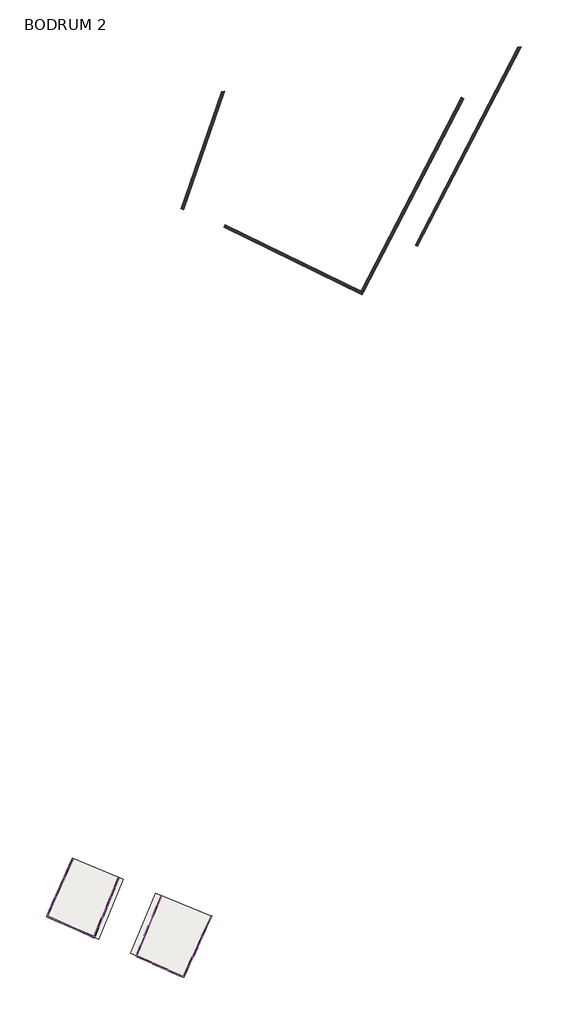
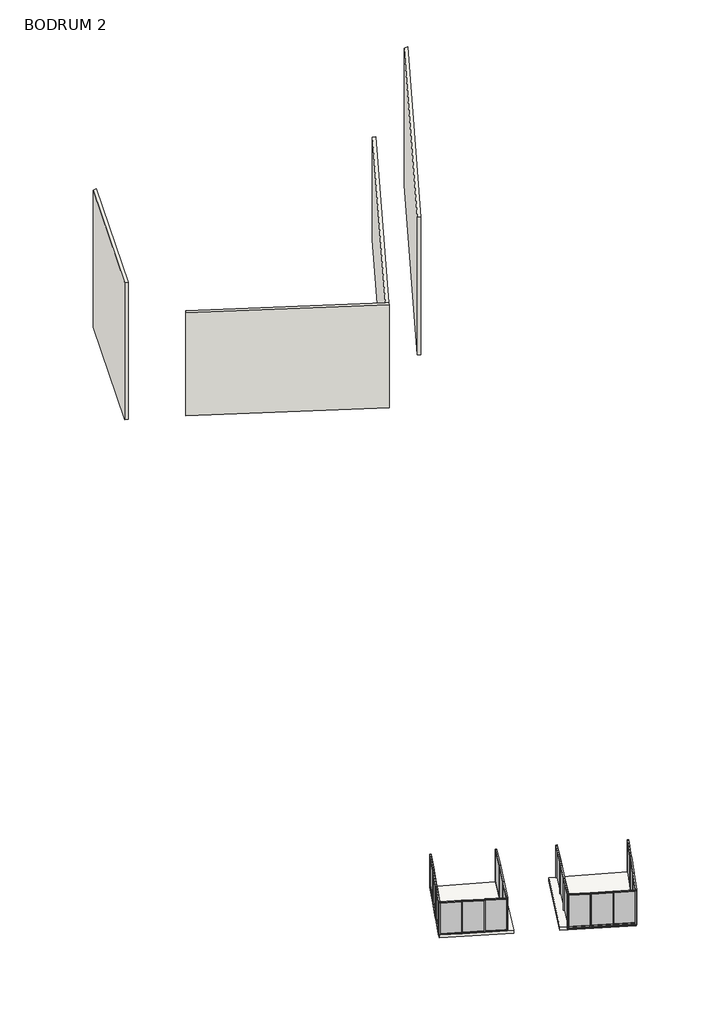
# One storey: 60 members, 18 plates, 4 walls, 1 slab.
"""IFC4 building model written with IfcOpenShell, lengths in millimetres."""

import ifcopenshell
import ifcopenshell.guid

model = None  # the IFC model being written
_history = None  # IfcOwnerHistory: only IFC2X3 demands one
_inside = {}  # id of a spatial element -> (the spatial element, [elements in it])
_under = {}  # id of a project, library or spatial element -> (it, [spatial elements below it])
_declared = {}  # id of a project -> (the project, [libraries it declares])
_typed = {}  # id of a type object -> (the type object, [elements of that type])
_made_of = {}  # id of a material, layer set ... -> (it, [elements and type objects made of it])


def new_model(schema):
    """Start an empty IFC model of exactly this schema.

    Asked for "IFC4X3", IfcOpenShell would pick the latest addendum, in which some entities
    have other attributes; the version numbers below select the first issue.
    IFC2X3 requires an IfcOwnerHistory on every rooted entity: one is made here for all.
    """
    global model, _history
    if schema == "IFC4X3":
        model = ifcopenshell.file(schema_version=(4, 3, 0, 0))
    else:
        model = ifcopenshell.file(schema=schema)
    _inside.clear()
    _under.clear()
    _declared.clear()
    _typed.clear()
    _made_of.clear()
    _history = None
    if model.schema == "IFC2X3":
        org = make("IfcOrganization", Name="unknown")
        user = make(
            "IfcPersonAndOrganization",
            ThePerson=make("IfcPerson", FamilyName="unknown"),
            TheOrganization=org,
        )
        app = make(
            "IfcApplication",
            ApplicationDeveloper=org,
            Version="unknown",
            ApplicationFullName="unknown",
            ApplicationIdentifier="unknown",
        )
        _history = make(
            "IfcOwnerHistory",
            OwningUser=user,
            OwningApplication=app,
            ChangeAction="ADDED",
            CreationDate=0,
        )
    return model


def make(cls, **values):
    """One entity of the class cls with the attributes given. An attribute that is None is left unset."""
    return model.create_entity(
        cls, **{name: value for name, value in values.items() if value is not None}
    )


def rooted(cls, **values):
    """An entity with a GlobalId (a new one), such as an element, a storey or a relation."""
    return make(cls, GlobalId=ifcopenshell.guid.new(), OwnerHistory=_history, **values)


def si_unit(unit_type, name, prefix=None):
    """IfcSIUnit, for example si_unit("LENGTHUNIT", "METRE", prefix="MILLI")."""
    return make("IfcSIUnit", UnitType=unit_type, Prefix=prefix, Name=name)


def assignment(units):
    """IfcUnitAssignment: the units of a project."""
    return None if units is None else make("IfcUnitAssignment", Units=units)


def point(xyz):
    """IfcCartesianPoint."""
    return None if xyz is None else make("IfcCartesianPoint", Coordinates=xyz)


def direction(xyz):
    """IfcDirection."""
    return None if xyz is None else make("IfcDirection", DirectionRatios=xyz)


def frame(location, z_axis=None, x_axis=None):
    """IfcAxis2Placement3D, a coordinate frame: its origin and axes. An axis left out is left unset."""
    return make(
        "IfcAxis2Placement3D",
        Location=point(location),
        Axis=direction(z_axis),
        RefDirection=direction(x_axis),
    )


def origin():
    """The frame at (0, 0, 0) with its axes left unset."""
    return frame((0.0, 0.0, 0.0))


def origin_with_axes():
    """The frame at (0, 0, 0) with the z axis (0, 0, 1) and the x axis (1, 0, 0) written out."""
    return frame((0.0, 0.0, 0.0), z_axis=(0.0, 0.0, 1.0), x_axis=(1.0, 0.0, 0.0))


def place(relative_to, where):
    """IfcLocalPlacement: puts the frame where relative to a parent placement (None: the world)."""
    return make(
        "IfcLocalPlacement", PlacementRelTo=relative_to, RelativePlacement=where
    )


def context(
    kind, dimensions, precision=None, world=None, true_north=None, identifier=None
):
    """IfcGeometricRepresentationContext, for example the 3D "Model" context."""
    return make(
        "IfcGeometricRepresentationContext",
        ContextIdentifier=identifier,
        ContextType=kind,
        CoordinateSpaceDimension=dimensions,
        Precision=precision,
        WorldCoordinateSystem=world,
        TrueNorth=true_north,
    )


def project(units=None, contexts=None):
    """IfcProject with its units and contexts."""
    return rooted(
        "IfcProject",
        Name="project",
        RepresentationContexts=contexts,
        UnitsInContext=assignment(units),
    )


def spatial(cls, under=None, at=None, **own):
    """A site, building, storey or space (cls), placed at a placement, below another one or the project."""
    s = rooted(cls, ObjectPlacement=at, **own)
    if under is not None:
        _under.setdefault(under.id(), (under, []))[1].append(s)
    return s


def polyline(points):
    """IfcPolyline through the points."""
    return make("IfcPolyline", Points=[point(p) for p in points])


def outline(outer, holes=None, kind="AREA"):
    """IfcArbitraryClosedProfileDef: a profile drawn as a closed curve; with holes, ...WithVoids."""
    if holes is None:
        return make("IfcArbitraryClosedProfileDef", ProfileType=kind, OuterCurve=outer)
    return make(
        "IfcArbitraryProfileDefWithVoids",
        ProfileType=kind,
        OuterCurve=outer,
        InnerCurves=holes,
    )


def extrude(swept, where, along, depth):
    """IfcExtrudedAreaSolid: the profile swept, set in the frame where, extruded along a direction by depth."""
    return make(
        "IfcExtrudedAreaSolid",
        SweptArea=swept,
        Position=where,
        ExtrudedDirection=direction(along),
        Depth=depth,
    )


def faces_of(points, faces, orient=None, outer=None):
    """IfcFace entities. A face is a list of loops; a loop is a list of indices into points, from 0.

    orient and outer hold one flag for each loop. By default every Orientation is true, the
    first loop of a face is its IfcFaceOuterBound and the others are IfcFaceBound.
    """
    made = []
    for i, loops in enumerate(faces):
        bounds = []
        for j, loop in enumerate(loops):
            is_outer = j == 0 if outer is None else outer[i][j]
            bounds.append(
                make(
                    "IfcFaceOuterBound" if is_outer else "IfcFaceBound",
                    Bound=make("IfcPolyLoop", Polygon=[points[k] for k in loop]),
                    Orientation=True if orient is None else orient[i][j],
                )
            )
        made.append(make("IfcFace", Bounds=bounds))
    return made


def faceted_brep(points, faces, orient=None, outer=None, voids=None):
    """IfcFacetedBrep: a solid bounded by flat faces; with voids (closed shells), ...WithVoids."""
    shared = [point(p) for p in points]
    hull = make("IfcClosedShell", CfsFaces=faces_of(shared, faces, orient, outer))
    if voids is None:
        return make("IfcFacetedBrep", Outer=hull)
    return make(
        "IfcFacetedBrepWithVoids",
        Outer=hull,
        Voids=[
            make(cls, CfsFaces=faces_of(shared, fs, o, b)) for cls, fs, o, b in voids
        ],
    )


def shape(context_of_items, identifier, shape_type, items):
    """IfcShapeRepresentation: the items that make up one representation, for example the "Body"."""
    return make(
        "IfcShapeRepresentation",
        ContextOfItems=context_of_items,
        RepresentationIdentifier=identifier,
        RepresentationType=shape_type,
        Items=items,
    )


def source(mapping_origin, context_of_items, identifier, shape_type, items):
    """IfcRepresentationMap: a shape defined once, which mapped items show again and again."""
    return make(
        "IfcRepresentationMap",
        MappingOrigin=mapping_origin,
        MappedRepresentation=shape(context_of_items, identifier, shape_type, items),
    )


def transform(
    local_origin,
    x_axis=None,
    y_axis=None,
    z_axis=None,
    scale=None,
    scale2=None,
    scale3=None,
    uniform=True,
):
    """IfcCartesianTransformationOperator3D, or its non-uniform kind. x_axis, y_axis, z_axis: its Axis1, 2, 3."""
    if uniform:
        return make(
            "IfcCartesianTransformationOperator3D",
            Axis1=direction(x_axis),
            Axis2=direction(y_axis),
            LocalOrigin=point(local_origin),
            Scale=scale,
            Axis3=direction(z_axis),
        )
    return make(
        "IfcCartesianTransformationOperator3DnonUniform",
        Axis1=direction(x_axis),
        Axis2=direction(y_axis),
        LocalOrigin=point(local_origin),
        Scale=scale,
        Axis3=direction(z_axis),
        Scale2=scale2,
        Scale3=scale3,
    )


def mapped(mapping_source, mapping_target):
    """IfcMappedItem: shows the shape of a source again, moved by a transform."""
    return make(
        "IfcMappedItem", MappingSource=mapping_source, MappingTarget=mapping_target
    )


def made_of(thing, what):
    """Note that an element or type object is made of a material, layer set ...; save() writes the relation."""
    if what is not None:
        _made_of.setdefault(what.id(), (what, []))[1].append(thing)
    return thing


def element(
    cls,
    number,
    at=None,
    inside=None,
    cuts=None,
    type_object=None,
    material=None,
    context=None,
    identifier="Body",
    shape_type=None,
    held_by="IfcProductDefinitionShape",
    body=None,
    shapes=None,
    **own,
):
    """One element of the class cls, such as IfcWall. Its Tag is "e" and its number.

    at: its placement. inside: the storey or other place that contains it. cuts: it is an
    opening in that element (IfcRelVoidsElement). A single representation is given by context,
    identifier, shape_type and body (its items); several are given by shapes. held_by: the class
    of the entity that holds the representations. save() writes the other relations.
    """
    e = rooted(cls, Tag="e%d" % number, ObjectPlacement=at, **own)
    if body is not None:
        shapes = [shape(context, identifier, shape_type, body)]
    if shapes is not None:
        e.Representation = make(held_by, Representations=shapes)
    if inside is not None:
        _inside.setdefault(inside.id(), (inside, []))[1].append(e)
    if cuts is not None:
        rooted(
            "IfcRelVoidsElement", RelatingBuildingElement=cuts, RelatedOpeningElement=e
        )
    if type_object is not None:
        _typed.setdefault(type_object.id(), (type_object, []))[1].append(e)
    return made_of(e, material)


def aggregate(whole, parts):
    """IfcRelAggregates: a whole, such as a stair, and the parts it consists of."""
    return rooted("IfcRelAggregates", RelatingObject=whole, RelatedObjects=parts)


def save(model, path):
    """Write the relations noted so far, then the file.

    IfcRelAggregates (storeys below a building ...), IfcRelContainedInSpatialStructure (elements
    in a storey), IfcRelDefinesByType, IfcRelAssociatesMaterial and IfcRelDeclares: one each for
    every whole, place, type object, material and project.
    """
    for whole, parts in _under.values():
        aggregate(whole, parts)
    for where, things in _inside.values():
        rooted(
            "IfcRelContainedInSpatialStructure",
            RelatedElements=things,
            RelatingStructure=where,
        )
    for kind, things in _typed.values():
        rooted("IfcRelDefinesByType", RelatedObjects=things, RelatingType=kind)
    for what, things in _made_of.values():
        rooted("IfcRelAssociatesMaterial", RelatedObjects=things, RelatingMaterial=what)
    for by, libraries in _declared.values():
        rooted("IfcRelDeclares", RelatingContext=by, RelatedDefinitions=libraries)
    model.write(path)


def rectangular_mullion_65_x_125mm_rectangular_245190dc(model_context):
    return source(origin(), model_context, "Body", "SweptSolid", [
        extrude(outline(polyline([(0.0, 62.5), (0.0, -62.5), (-65.0, -62.5), (-65.0, 62.5), (0.0, 62.5)])), frame((0.0, 0.0, -2244.830414), z_axis=(0.0, 0.0, 1.0), x_axis=(1.0, 0.0, 0.0)), (0.0, 0.0, 1.0), 2244.830414),
    ])


def rectangular_mullion_65_x_125mm_rectangular_478791df(model_context):
    return source(origin(), model_context, "Body", "SweptSolid", [
        extrude(outline(polyline([(0.0, 62.5), (0.0, -62.5), (-65.0, -62.5), (-65.0, 62.5), (0.0, 62.5)])), frame((0.0, 0.0, -2277.3304137), z_axis=(0.0, 0.0, 1.0), x_axis=(1.0, 0.0, 0.0)), (0.0, 0.0, 1.0), 2277.3304137),
    ])


def rectangular_mullion_65_x_125mm_rectangular_36adfa9f(model_context):
    return source(origin(), model_context, "Body", "SweptSolid", [
        extrude(outline(polyline([(0.0, 62.5), (0.0, -62.5), (-65.0, -62.5), (-65.0, 62.5), (0.0, 62.5)])), frame((0.0, 0.0, -1809.1666668), z_axis=(0.0, 0.0, 1.0), x_axis=(1.0, 0.0, 0.0)), (0.0, 0.0, 1.0), 1809.1666668),
    ])


def rectangular_mullion_65_x_125mm_rectangular_c7ba065f(model_context):
    return source(origin(), model_context, "Body", "SweptSolid", [
        extrude(outline(polyline([(0.0, 62.5), (0.0, -62.5), (-65.0, -62.5), (-65.0, 62.5), (0.0, 62.5)])), frame((0.0, 0.0, -1841.6666665), z_axis=(0.0, 0.0, 1.0), x_axis=(1.0, 0.0, 0.0)), (0.0, 0.0, 1.0), 1841.6666665),
    ])


def rectangular_mullion_65_x_125mm_rectangular_4f7d984b(model_context):
    return source(origin(), model_context, "Body", "SweptSolid", [
        extrude(outline(polyline([(0.0, 62.5), (0.0, -62.5), (-65.0, -62.5), (-65.0, 62.5), (0.0, 62.5)])), frame((0.0, 0.0, -2291.9433297), z_axis=(0.0, 0.0, 1.0), x_axis=(1.0, 0.0, 0.0)), (0.0, 0.0, 1.0), 2291.9433297),
    ])


def rectangular_mullion_65_x_125mm_rectangular_64dbaea3(model_context):
    return source(origin(), model_context, "Body", "SweptSolid", [
        extrude(outline(polyline([(0.0, 62.5), (0.0, -62.5), (-65.0, -62.5), (-65.0, 62.5), (0.0, 62.5)])), frame((0.0, 0.0, -2324.4433294), z_axis=(0.0, 0.0, 1.0), x_axis=(1.0, 0.0, 0.0)), (0.0, 0.0, 1.0), 2324.4433294),
    ])


def rectangular_mullion_65_x_125mm_rectangular_bddaf145(model_context):
    return source(origin(), model_context, "Body", "SweptSolid", [
        extrude(outline(polyline([(32.5, 62.5), (32.5, -62.5), (-32.5, -62.5), (-32.5, 62.5), (32.5, 62.5)])), frame((0.0, 0.0, -3300.0), z_axis=(0.0, 0.0, 1.0), x_axis=(1.0, 0.0, 0.0)), (0.0, 0.0, 1.0), 3300.0),
    ])


def rectangular_mullion_65_x_125mm_rectangular_6bff5ffe(model_context):
    return source(origin(), model_context, "Body", "SweptSolid", [
        extrude(outline(polyline([(0.0, 62.5), (0.0, -62.5), (-65.0, -62.5), (-65.0, 62.5), (0.0, 62.5)])), frame((0.0, 0.0, -3300.0), z_axis=(0.0, 0.0, 1.0), x_axis=(1.0, 0.0, 0.0)), (0.0, 0.0, 1.0), 3300.0),
    ])


def rectangular_mullion_65_x_125mm_rectangular_eddbc5d6(model_context):
    return source(origin(), model_context, "Body", "SweptSolid", [
        extrude(outline(polyline([(0.0, 62.5), (0.0, -62.5), (-65.0, -62.5), (-65.0, 62.5), (0.0, 62.5)])), frame((0.0, 0.0, -2323.142254), z_axis=(0.0, 0.0, 1.0), x_axis=(1.0, 0.0, 0.0)), (0.0, 0.0, 1.0), 2323.142254),
    ])


def rectangular_mullion_65_x_125mm_rectangular_617b4e42(model_context):
    return source(origin(), model_context, "Body", "SweptSolid", [
        extrude(outline(polyline([(0.0, 62.5), (0.0, -62.5), (-65.0, -62.5), (-65.0, 62.5), (0.0, 62.5)])), frame((0.0, 0.0, -2355.6422537), z_axis=(0.0, 0.0, 1.0), x_axis=(1.0, 0.0, 0.0)), (0.0, 0.0, 1.0), 2355.6422537),
    ])


def rectangular_mullion_65_x_125mm_rectangular_c6a61499(model_context):
    return source(origin(), model_context, "Body", "SweptSolid", [
        extrude(outline(polyline([(32.5, 62.5), (32.5, -62.5), (-32.5, -62.5), (-32.5, 62.5), (32.5, 62.5)])), frame((0.0, 0.0, -3500.0), z_axis=(0.0, 0.0, 1.0), x_axis=(1.0, 0.0, 0.0)), (0.0, 0.0, 1.0), 3500.0),
    ])


def rectangular_mullion_65_x_125mm_rectangular_efb59fec(model_context):
    return source(origin(), model_context, "Body", "SweptSolid", [
        extrude(outline(polyline([(0.0, 62.5), (0.0, -62.5), (-65.0, -62.5), (-65.0, 62.5), (0.0, 62.5)])), frame((0.0, 0.0, -3500.0), z_axis=(0.0, 0.0, 1.0), x_axis=(1.0, 0.0, 0.0)), (0.0, 0.0, 1.0), 3500.0),
    ])


def rectangular_mullion_65_x_125mm_rectangular_567d2977(model_context):
    return source(origin(), model_context, "Body", "SweptSolid", [
        extrude(outline(polyline([(0.0, 62.5), (0.0, -62.5), (-65.0, -62.5), (-65.0, 62.5), (0.0, 62.5)])), frame((0.0, 0.0, -1811.8827626), z_axis=(0.0, 0.0, 1.0), x_axis=(1.0, 0.0, 0.0)), (0.0, 0.0, 1.0), 1811.8827626),
    ])


def rectangular_mullion_65_x_125mm_rectangular_abf36099(model_context):
    return source(origin(), model_context, "Body", "SweptSolid", [
        extrude(outline(polyline([(0.0, 62.5), (0.0, -62.5), (-65.0, -62.5), (-65.0, 62.5), (0.0, 62.5)])), frame((0.0, 0.0, -1844.3827623), z_axis=(0.0, 0.0, 1.0), x_axis=(1.0, 0.0, 0.0)), (0.0, 0.0, 1.0), 1844.3827623),
    ])


def rectangular_mullion_65_x_125mm_rectangular_944d97ce(model_context):
    return source(origin(), model_context, "Body", "SweptSolid", [
        extrude(outline(polyline([(0.0, 62.5), (0.0, -62.5), (-65.0, -62.5), (-65.0, 62.5), (0.0, 62.5)])), frame((0.0, 0.0, -2373.0683182), z_axis=(0.0, 0.0, 1.0), x_axis=(1.0, 0.0, 0.0)), (0.0, 0.0, 1.0), 2373.0683182),
    ])


def rectangular_mullion_65_x_125mm_rectangular_8233692a(model_context):
    return source(origin(), model_context, "Body", "SweptSolid", [
        extrude(outline(polyline([(0.0, 62.5), (0.0, -62.5), (-65.0, -62.5), (-65.0, 62.5), (0.0, 62.5)])), frame((0.0, 0.0, -2405.5683179), z_axis=(0.0, 0.0, 1.0), x_axis=(1.0, 0.0, 0.0)), (0.0, 0.0, 1.0), 2405.5683179),
    ])


def system_panel_glazed_19379390(model_context):
    return source(origin(), model_context, "Body", "SweptSolid", [
        extrude(outline(polyline([(1122.415207, 24.5), (-1122.415207, 24.5), (-1122.415207, 49.5), (1122.415207, 49.5), (1122.415207, 24.5)])), origin_with_axes(), (0.0, 0.0, 1.0), 3170.0),
    ])


def system_panel_glazed_0a1ee489(model_context):
    return source(origin(), model_context, "Body", "SweptSolid", [
        extrude(outline(polyline([(1138.6652068, 24.5), (-1138.6652068, 24.5), (-1138.6652068, 49.5), (1138.6652068, 49.5), (1138.6652068, 24.5)])), origin_with_axes(), (0.0, 0.0, 1.0), 3170.0),
    ])


def system_panel_glazed_d1c08d78(model_context):
    return source(origin(), model_context, "Body", "SweptSolid", [
        extrude(outline(polyline([(904.5833334, 24.5), (-904.5833334, 24.5), (-904.5833334, 49.5), (904.5833334, 49.5), (904.5833334, 24.5)])), origin_with_axes(), (0.0, 0.0, 1.0), 3170.0),
    ])


def system_panel_glazed_7daaf864(model_context):
    return source(origin(), model_context, "Body", "SweptSolid", [
        extrude(outline(polyline([(920.8333332, 24.5), (-920.8333332, 24.5), (-920.8333332, 49.5), (920.8333332, 49.5), (920.8333332, 24.5)])), origin_with_axes(), (0.0, 0.0, 1.0), 3170.0),
    ])


def system_panel_glazed_4d4608c9(model_context):
    return source(origin(), model_context, "Body", "SweptSolid", [
        extrude(outline(polyline([(1145.9716649, 24.5), (-1145.9716649, 24.5), (-1145.9716649, 49.5), (1145.9716649, 49.5), (1145.9716649, 24.5)])), origin_with_axes(), (0.0, 0.0, 1.0), 3170.0),
    ])


def system_panel_glazed_4b2262bb(model_context):
    return source(origin(), model_context, "Body", "SweptSolid", [
        extrude(outline(polyline([(1162.2216647, 24.5), (-1162.2216647, 24.5), (-1162.2216647, 49.5), (1162.2216647, 49.5), (1162.2216647, 24.5)])), origin_with_axes(), (0.0, 0.0, 1.0), 3170.0),
    ])


def system_panel_glazed_6ba5d601(model_context):
    return source(origin(), model_context, "Body", "SweptSolid", [
        extrude(outline(polyline([(1161.571127, 24.5), (-1161.571127, 24.5), (-1161.571127, 49.5), (1161.571127, 49.5), (1161.571127, 24.5)])), origin_with_axes(), (0.0, 0.0, 1.0), 3370.0),
    ])


def system_panel_glazed_15c79043(model_context):
    return source(origin(), model_context, "Body", "SweptSolid", [
        extrude(outline(polyline([(1177.8211268, 24.5), (-1177.8211268, 24.5), (-1177.8211268, 49.5), (1177.8211268, 49.5), (1177.8211268, 24.5)])), origin_with_axes(), (0.0, 0.0, 1.0), 3370.0),
    ])


def system_panel_glazed_6ec36b42(model_context):
    return source(origin(), model_context, "Body", "SweptSolid", [
        extrude(outline(polyline([(905.9413813, 24.5), (-905.9413813, 24.5), (-905.9413813, 49.5), (905.9413813, 49.5), (905.9413813, 24.5)])), origin_with_axes(), (0.0, 0.0, 1.0), 3370.0),
    ])


def system_panel_glazed_f294eff5(model_context):
    return source(origin(), model_context, "Body", "SweptSolid", [
        extrude(outline(polyline([(922.1913812, 24.5), (-922.1913812, 24.5), (-922.1913812, 49.5), (922.1913812, 49.5), (922.1913812, 24.5)])), origin_with_axes(), (0.0, 0.0, 1.0), 3370.0),
    ])


def system_panel_glazed_e4114e99(model_context):
    return source(origin(), model_context, "Body", "SweptSolid", [
        extrude(outline(polyline([(1186.5341591, 24.5), (-1186.5341591, 24.5), (-1186.5341591, 49.5), (1186.5341591, 49.5), (1186.5341591, 24.5)])), origin_with_axes(), (0.0, 0.0, 1.0), 3370.0),
    ])


def system_panel_glazed_ce7d9ee4(model_context):
    return source(origin(), model_context, "Body", "SweptSolid", [
        extrude(outline(polyline([(1202.784159, 24.5), (-1202.784159, 24.5), (-1202.784159, 49.5), (1202.784159, 49.5), (1202.784159, 24.5)])), origin_with_axes(), (0.0, 0.0, 1.0), 3370.0),
    ])


model = new_model("IFC4")

# Units and contexts
model_context = context("Model", 3, world=origin())
ifc_project = project(units=[si_unit("LENGTHUNIT", "METRE", prefix="MILLI")], contexts=[model_context])

# Site, building, storey
site = spatial("IfcSite", under=ifc_project)
building = spatial("IfcBuilding", under=site)
storey = spatial("IfcBuildingStorey", under=building, Name="BODRUM 2", Elevation=-7000.0)

# Members
placement = place(None, origin())
rectangular_mullion_65_x_125mm_rectangular_shape = rectangular_mullion_65_x_125mm_rectangular_245190dc(model_context)
element("IfcMember", 1, ObjectType="Rectangular Mullion : 65 x 125mm rectangular", at=placement, inside=storey, context=model_context, shape_type="MappedRepresentation", body=[
    mapped(rectangular_mullion_65_x_125mm_rectangular_shape, transform((-105369.8109554, 121836.1504415, -3500.0), x_axis=(0.0, 0.0, 1.0), y_axis=(-0.9138108396305767, 0.4061400612764768, 0.0), z_axis=(-0.4061400612764768, -0.9138108396305767, 0.0))),
])
element("IfcMember", 2, ObjectType="Rectangular Mullion : 65 x 125mm rectangular", at=placement, inside=storey, context=model_context, shape_type="MappedRepresentation", body=[
    mapped(rectangular_mullion_65_x_125mm_rectangular_shape, transform((-103480.3820718, 126087.3454336, -3500.0), x_axis=(0.0, 0.0, 1.0), y_axis=(-0.9138108396305767, 0.4061400612764768, 0.0), z_axis=(-0.4061400612764768, -0.9138108396305767, 0.0))),
])
rectangular_mullion_65_x_125mm_rectangular_2_shape = rectangular_mullion_65_x_125mm_rectangular_478791df(model_context)
element("IfcMember", 3, ObjectType="Rectangular Mullion : 65 x 125mm rectangular", at=placement, inside=storey, context=model_context, shape_type="MappedRepresentation", body=[
    mapped(rectangular_mullion_65_x_125mm_rectangular_2_shape, transform((-104431.6962895, 123946.8985115, -3500.0), x_axis=(0.0, 0.0, 1.0), y_axis=(-0.913810839630577, 0.40614006127647634, 0.0), z_axis=(-0.40614006127647634, -0.913810839630577, 0.0))),
])
element("IfcMember", 4, ObjectType="Rectangular Mullion : 65 x 125mm rectangular", at=placement, inside=storey, context=model_context, shape_type="MappedRepresentation", body=[
    mapped(rectangular_mullion_65_x_125mm_rectangular_shape, transform((-102568.6665099, 128138.695799, -6800.0), x_axis=(0.0, 0.0, -1.0), y_axis=(-0.9138108396305767, 0.4061400612764768, 0.0), z_axis=(0.4061400612764768, 0.9138108396305767, 0.0))),
])
element("IfcMember", 5, ObjectType="Rectangular Mullion : 65 x 125mm rectangular", at=placement, inside=storey, context=model_context, shape_type="MappedRepresentation", body=[
    mapped(rectangular_mullion_65_x_125mm_rectangular_shape, transform((-104458.0953935, 123887.500807, -6800.0), x_axis=(0.0, 0.0, -1.0), y_axis=(-0.9138108396305767, 0.4061400612764768, 0.0), z_axis=(0.4061400612764768, 0.9138108396305767, 0.0))),
])
element("IfcMember", 6, ObjectType="Rectangular Mullion : 65 x 125mm rectangular", at=placement, inside=storey, context=model_context, shape_type="MappedRepresentation", body=[
    mapped(rectangular_mullion_65_x_125mm_rectangular_2_shape, transform((-103506.7811758, 126027.947729, -6800.0), x_axis=(0.0, 0.0, -1.0), y_axis=(-0.913810839630577, 0.40614006127647634, 0.0), z_axis=(0.40614006127647634, 0.913810839630577, 0.0))),
])
rectangular_mullion_65_x_125mm_rectangular_3_shape = rectangular_mullion_65_x_125mm_rectangular_36adfa9f(model_context)
element("IfcMember", 7, ObjectType="Rectangular Mullion : 65 x 125mm rectangular", at=placement, inside=storey, context=model_context, shape_type="MappedRepresentation", body=[
    mapped(rectangular_mullion_65_x_125mm_rectangular_3_shape, transform((-100228.6097613, 119480.0306904, -3500.0), x_axis=(0.0, 0.0, 1.0), y_axis=(-0.4061400612764708, -0.9138108396305795, 0.0), z_axis=(0.9138108396305794, -0.40614006127647073, 0.0))),
])
element("IfcMember", 8, ObjectType="Rectangular Mullion : 65 x 125mm rectangular", at=placement, inside=storey, context=model_context, shape_type="MappedRepresentation", body=[
    mapped(rectangular_mullion_65_x_125mm_rectangular_3_shape, transform((-103683.576244, 121015.5785721, -3500.0), x_axis=(0.0, 0.0, 1.0), y_axis=(-0.4061400612764708, -0.9138108396305795, 0.0), z_axis=(0.9138108396305794, -0.40614006127647073, 0.0))),
])
rectangular_mullion_65_x_125mm_rectangular_4_shape = rectangular_mullion_65_x_125mm_rectangular_c7ba065f(model_context)
element("IfcMember", 9, ObjectType="Rectangular Mullion : 65 x 125mm rectangular", at=placement, inside=storey, context=model_context, shape_type="MappedRepresentation", body=[
    mapped(rectangular_mullion_65_x_125mm_rectangular_4_shape, transform((-101941.2435767, 120241.2048553, -3500.0), x_axis=(0.0, 0.0, 1.0), y_axis=(-0.4061400612764777, -0.9138108396305764, 0.0), z_axis=(0.9138108396305764, -0.4061400612764777, 0.0))),
])
element("IfcMember", 10, ObjectType="Rectangular Mullion : 65 x 125mm rectangular", at=placement, inside=storey, context=model_context, shape_type="MappedRepresentation", body=[
    mapped(rectangular_mullion_65_x_125mm_rectangular_3_shape, transform((-105336.8123548, 121750.353633, -6800.0), x_axis=(0.0, 0.0, -1.0), y_axis=(-0.4061400612764708, -0.9138108396305795, 0.0), z_axis=(-0.9138108396305794, 0.40614006127647073, 0.0))),
])
element("IfcMember", 11, ObjectType="Rectangular Mullion : 65 x 125mm rectangular", at=placement, inside=storey, context=model_context, shape_type="MappedRepresentation", body=[
    mapped(rectangular_mullion_65_x_125mm_rectangular_3_shape, transform((-101881.8458721, 120214.8057513, -6800.0), x_axis=(0.0, 0.0, -1.0), y_axis=(-0.4061400612764708, -0.9138108396305795, 0.0), z_axis=(-0.9138108396305794, 0.40614006127647073, 0.0))),
])
element("IfcMember", 12, ObjectType="Rectangular Mullion : 65 x 125mm rectangular", at=placement, inside=storey, context=model_context, shape_type="MappedRepresentation", body=[
    mapped(rectangular_mullion_65_x_125mm_rectangular_4_shape, transform((-103624.1785395, 120989.1794681, -6800.0), x_axis=(0.0, 0.0, -1.0), y_axis=(-0.4061400612764777, -0.9138108396305764, 0.0), z_axis=(-0.9138108396305764, 0.4061400612764777, 0.0))),
])
rectangular_mullion_65_x_125mm_rectangular_5_shape = rectangular_mullion_65_x_125mm_rectangular_4f7d984b(model_context)
element("IfcMember", 13, ObjectType="Rectangular Mullion : 65 x 125mm rectangular", at=placement, inside=storey, context=model_context, shape_type="MappedRepresentation", body=[
    mapped(rectangular_mullion_65_x_125mm_rectangular_5_shape, transform((-97448.0777742, 126015.0891338, -3500.0), x_axis=(0.0, 0.0, 1.0), y_axis=(0.9237157161132051, -0.3830786809592367, 0.0), z_axis=(0.3830786809592367, 0.9237157161132051, 0.0))),
])
element("IfcMember", 14, ObjectType="Rectangular Mullion : 65 x 125mm rectangular", at=placement, inside=storey, context=model_context, shape_type="MappedRepresentation", body=[
    mapped(rectangular_mullion_65_x_125mm_rectangular_5_shape, transform((-99266.3173149, 121630.7771821, -3500.0), x_axis=(0.0, 0.0, 1.0), y_axis=(0.9237157161132051, -0.3830786809592367, 0.0), z_axis=(0.3830786809592367, 0.9237157161132051, 0.0))),
])
rectangular_mullion_65_x_125mm_rectangular_6_shape = rectangular_mullion_65_x_125mm_rectangular_64dbaea3(model_context)
element("IfcMember", 15, ObjectType="Rectangular Mullion : 65 x 125mm rectangular", at=placement, inside=storey, context=model_context, shape_type="MappedRepresentation", body=[
    mapped(rectangular_mullion_65_x_125mm_rectangular_6_shape, transform((-98350.972516, 123837.9435382, -3500.0), x_axis=(0.0, 0.0, 1.0), y_axis=(0.9237157161132034, -0.383078680959241, 0.0), z_axis=(0.383078680959241, 0.9237157161132034, 0.0))),
])
element("IfcMember", 16, ObjectType="Rectangular Mullion : 65 x 125mm rectangular", at=placement, inside=storey, context=model_context, shape_type="MappedRepresentation", body=[
    mapped(rectangular_mullion_65_x_125mm_rectangular_5_shape, transform((-100144.3119424, 119513.673108, -6800.0), x_axis=(0.0, 0.0, -1.0), y_axis=(0.9237157161132051, -0.3830786809592367, 0.0), z_axis=(-0.3830786809592367, -0.9237157161132051, 0.0))),
])
element("IfcMember", 17, ObjectType="Rectangular Mullion : 65 x 125mm rectangular", at=placement, inside=storey, context=model_context, shape_type="MappedRepresentation", body=[
    mapped(rectangular_mullion_65_x_125mm_rectangular_5_shape, transform((-98326.0724018, 123897.9850597, -6800.0), x_axis=(0.0, 0.0, -1.0), y_axis=(0.9237157161132051, -0.3830786809592367, 0.0), z_axis=(-0.3830786809592367, -0.9237157161132051, 0.0))),
])
element("IfcMember", 18, ObjectType="Rectangular Mullion : 65 x 125mm rectangular", at=placement, inside=storey, context=model_context, shape_type="MappedRepresentation", body=[
    mapped(rectangular_mullion_65_x_125mm_rectangular_6_shape, transform((-99241.4172006, 121690.8187036, -6800.0), x_axis=(0.0, 0.0, -1.0), y_axis=(0.9237157161132034, -0.383078680959241, 0.0), z_axis=(-0.383078680959241, -0.9237157161132034, 0.0))),
])
rectangular_mullion_65_x_125mm_rectangular_7_shape = rectangular_mullion_65_x_125mm_rectangular_bddaf145(model_context)
element("IfcMember", 19, ObjectType="Rectangular Mullion : 65 x 125mm rectangular", at=placement, inside=storey, context=model_context, shape_type="MappedRepresentation", body=[
    mapped(rectangular_mullion_65_x_125mm_rectangular_7_shape, transform((-103493.5816238, 126057.6465813, -6800.0), x_axis=(-0.4061400612764766, -0.9138108396305769, 0.0), y_axis=(-0.9138108396305769, 0.4061400612764766, 0.0), z_axis=(0.0, 0.0, -1.0))),
])
element("IfcMember", 20, ObjectType="Rectangular Mullion : 65 x 125mm rectangular", at=placement, inside=storey, context=model_context, shape_type="MappedRepresentation", body=[
    mapped(rectangular_mullion_65_x_125mm_rectangular_7_shape, transform((-104444.8958415, 123917.1996592, -6800.0), x_axis=(-0.4061400612764766, -0.9138108396305769, 0.0), y_axis=(-0.9138108396305769, 0.4061400612764766, 0.0), z_axis=(0.0, 0.0, -1.0))),
])
element("IfcMember", 21, ObjectType="Rectangular Mullion : 65 x 125mm rectangular", at=placement, inside=storey, context=model_context, shape_type="MappedRepresentation", body=[
    mapped(rectangular_mullion_65_x_125mm_rectangular_7_shape, transform((-103653.8773917, 121002.3790201, -6800.0), x_axis=(0.9138108396305787, -0.40614006127647245, 0.0), y_axis=(-0.40614006127647245, -0.9138108396305787, 0.0), z_axis=(0.0, 0.0, -1.0))),
])
element("IfcMember", 22, ObjectType="Rectangular Mullion : 65 x 125mm rectangular", at=placement, inside=storey, context=model_context, shape_type="MappedRepresentation", body=[
    mapped(rectangular_mullion_65_x_125mm_rectangular_7_shape, transform((-101911.5447244, 120228.0053033, -6800.0), x_axis=(0.9138108396305787, -0.40614006127647245, 0.0), y_axis=(-0.40614006127647245, -0.9138108396305787, 0.0), z_axis=(0.0, 0.0, -1.0))),
])
element("IfcMember", 23, ObjectType="Rectangular Mullion : 65 x 125mm rectangular", at=placement, inside=storey, context=model_context, shape_type="MappedRepresentation", body=[
    mapped(rectangular_mullion_65_x_125mm_rectangular_7_shape, transform((-99253.8672577, 121660.7979428, -6800.0), x_axis=(0.3830786809592386, 0.9237157161132044, 0.0), y_axis=(0.9237157161132044, -0.3830786809592386, 0.0), z_axis=(0.0, 0.0, -1.0))),
])
element("IfcMember", 24, ObjectType="Rectangular Mullion : 65 x 125mm rectangular", at=placement, inside=storey, context=model_context, shape_type="MappedRepresentation", body=[
    mapped(rectangular_mullion_65_x_125mm_rectangular_7_shape, transform((-98338.5224589, 123867.964299, -6800.0), x_axis=(0.3830786809592386, 0.9237157161132044, 0.0), y_axis=(0.9237157161132044, -0.3830786809592386, 0.0), z_axis=(0.0, 0.0, -1.0))),
])
rectangular_mullion_65_x_125mm_rectangular_8_shape = rectangular_mullion_65_x_125mm_rectangular_6bff5ffe(model_context)
element("IfcMember", 25, ObjectType="Rectangular Mullion : 65 x 125mm rectangular", at=placement, inside=storey, context=model_context, shape_type="MappedRepresentation", body=[
    mapped(rectangular_mullion_65_x_125mm_rectangular_8_shape, transform((-105396.2100594, 121776.7527369, -6800.0), x_axis=(-0.4061400612764766, -0.9138108396305769, 0.0), y_axis=(-0.9138108396305769, 0.4061400612764766, 0.0), z_axis=(0.0, 0.0, -1.0))),
])
element("IfcMember", 26, ObjectType="Rectangular Mullion : 65 x 125mm rectangular", at=placement, inside=storey, context=model_context, shape_type="MappedRepresentation", body=[
    mapped(rectangular_mullion_65_x_125mm_rectangular_8_shape, transform((-100169.2120567, 119453.6315864, -6800.0), x_axis=(0.9138108396305787, -0.40614006127647245, 0.0), y_axis=(-0.40614006127647245, -0.9138108396305787, 0.0), z_axis=(0.0, 0.0, -1.0))),
])
element("IfcMember", 27, ObjectType="Rectangular Mullion : 65 x 125mm rectangular", at=placement, inside=storey, context=model_context, shape_type="MappedRepresentation", body=[
    mapped(rectangular_mullion_65_x_125mm_rectangular_8_shape, transform((-97423.1776599, 126075.1306554, -6800.0), x_axis=(0.3830786809592386, 0.9237157161132044, 0.0), y_axis=(0.9237157161132044, -0.3830786809592386, 0.0), z_axis=(0.0, 0.0, -1.0))),
])
element("IfcMember", 28, ObjectType="Rectangular Mullion : 65 x 125mm rectangular", at=placement, inside=storey, context=model_context, shape_type="MappedRepresentation", body=[
    mapped(rectangular_mullion_65_x_125mm_rectangular_8_shape, transform((-102542.2674059, 128198.0935036, -3500.0), x_axis=(0.4061400612764766, 0.9138108396305769, 0.0), y_axis=(-0.9138108396305769, 0.4061400612764766, 0.0), z_axis=(0.0, 0.0, 1.0))),
])
element("IfcMember", 29, ObjectType="Rectangular Mullion : 65 x 125mm rectangular", at=placement, inside=storey, context=model_context, shape_type="MappedRepresentation", body=[
    mapped(rectangular_mullion_65_x_125mm_rectangular_8_shape, transform((-105396.2100594, 121776.7527369, -3500.0), x_axis=(-0.9138108396305787, 0.40614006127647245, 0.0), y_axis=(-0.40614006127647245, -0.9138108396305787, 0.0), z_axis=(0.0, 0.0, 1.0))),
])
element("IfcMember", 30, ObjectType="Rectangular Mullion : 65 x 125mm rectangular", at=placement, inside=storey, context=model_context, shape_type="MappedRepresentation", body=[
    mapped(rectangular_mullion_65_x_125mm_rectangular_8_shape, transform((-100169.2120567, 119453.6315864, -3500.0), x_axis=(-0.3830786809592386, -0.9237157161132044, 0.0), y_axis=(0.9237157161132044, -0.3830786809592386, 0.0), z_axis=(0.0, 0.0, 1.0))),
])
rectangular_mullion_65_x_125mm_rectangular_9_shape = rectangular_mullion_65_x_125mm_rectangular_eddbc5d6(model_context)
element("IfcMember", 31, ObjectType="Rectangular Mullion : 65 x 125mm rectangular", at=placement, inside=storey, context=model_context, shape_type="MappedRepresentation", body=[
    mapped(rectangular_mullion_65_x_125mm_rectangular_9_shape, transform((-95482.4079965, 117441.7060529, -3500.0), x_axis=(0.0, 0.0, 1.0), y_axis=(-0.9237157161132044, 0.38307868095923847, 0.0), z_axis=(-0.38307868095923847, -0.9237157161132044, 0.0))),
])
element("IfcMember", 32, ObjectType="Rectangular Mullion : 65 x 125mm rectangular", at=placement, inside=storey, context=model_context, shape_type="MappedRepresentation", body=[
    mapped(rectangular_mullion_65_x_125mm_rectangular_9_shape, transform((-93640.2651703, 121883.655878, -3500.0), x_axis=(0.0, 0.0, 1.0), y_axis=(-0.9237157161132055, 0.38307868095923603, 0.0), z_axis=(-0.38307868095923603, -0.9237157161132055, 0.0))),
])
rectangular_mullion_65_x_125mm_rectangular_10_shape = rectangular_mullion_65_x_125mm_rectangular_617b4e42(model_context)
element("IfcMember", 33, ObjectType="Rectangular Mullion : 65 x 125mm rectangular", at=placement, inside=storey, context=model_context, shape_type="MappedRepresentation", body=[
    mapped(rectangular_mullion_65_x_125mm_rectangular_10_shape, transform((-94567.5616119, 119647.6705852, -3500.0), x_axis=(0.0, 0.0, 1.0), y_axis=(-0.9237157161132041, 0.38307868095923925, 0.0), z_axis=(-0.3830786809592392, -0.923715716113204, 0.0))),
])
element("IfcMember", 34, ObjectType="Rectangular Mullion : 65 x 125mm rectangular", at=placement, inside=storey, context=model_context, shape_type="MappedRepresentation", body=[
    mapped(rectangular_mullion_65_x_125mm_rectangular_9_shape, transform((-92750.3188999, 124029.5788888, -7000.0), x_axis=(0.0, 0.0, -1.0), y_axis=(-0.9237157161132055, 0.38307868095923603, 0.0), z_axis=(0.38307868095923603, 0.9237157161132055, 0.0))),
])
element("IfcMember", 35, ObjectType="Rectangular Mullion : 65 x 125mm rectangular", at=placement, inside=storey, context=model_context, shape_type="MappedRepresentation", body=[
    mapped(rectangular_mullion_65_x_125mm_rectangular_9_shape, transform((-94592.4617261, 119587.6290637, -7000.0), x_axis=(0.0, 0.0, -1.0), y_axis=(-0.9237157161132044, 0.38307868095923847, 0.0), z_axis=(0.38307868095923847, 0.9237157161132044, 0.0))),
])
element("IfcMember", 36, ObjectType="Rectangular Mullion : 65 x 125mm rectangular", at=placement, inside=storey, context=model_context, shape_type="MappedRepresentation", body=[
    mapped(rectangular_mullion_65_x_125mm_rectangular_10_shape, transform((-93665.1652845, 121823.6143565, -7000.0), x_axis=(0.0, 0.0, -1.0), y_axis=(-0.9237157161132041, 0.38307868095923925, 0.0), z_axis=(0.3830786809592392, 0.923715716113204, 0.0))),
])
rectangular_mullion_65_x_125mm_rectangular_11_shape = rectangular_mullion_65_x_125mm_rectangular_c6a61499(model_context)
element("IfcMember", 37, ObjectType="Rectangular Mullion : 65 x 125mm rectangular", at=placement, inside=storey, context=model_context, shape_type="MappedRepresentation", body=[
    mapped(rectangular_mullion_65_x_125mm_rectangular_11_shape, transform((-93652.7152274, 121853.6351173, -7000.0), x_axis=(-0.3830786809592379, -0.9237157161132047, 0.0), y_axis=(-0.9237157161132047, 0.3830786809592379, 0.0), z_axis=(0.0, 0.0, -1.0))),
])
element("IfcMember", 38, ObjectType="Rectangular Mullion : 65 x 125mm rectangular", at=placement, inside=storey, context=model_context, shape_type="MappedRepresentation", body=[
    mapped(rectangular_mullion_65_x_125mm_rectangular_11_shape, transform((-94580.011669, 119617.6498245, -7000.0), x_axis=(-0.3830786809592379, -0.9237157161132047, 0.0), y_axis=(-0.9237157161132047, 0.3830786809592379, 0.0), z_axis=(0.0, 0.0, -1.0))),
])
element("IfcMember", 39, ObjectType="Rectangular Mullion : 65 x 125mm rectangular", at=placement, inside=storey, context=model_context, shape_type="MappedRepresentation", body=[
    mapped(rectangular_mullion_65_x_125mm_rectangular_11_shape, transform((-93762.4934452, 116606.1876992, -7000.0), x_axis=(0.9138108396305739, -0.40614006127648333, 0.0), y_axis=(-0.40614006127648333, -0.9138108396305739, 0.0), z_axis=(0.0, 0.0, -1.0))),
])
element("IfcMember", 40, ObjectType="Rectangular Mullion : 65 x 125mm rectangular", at=placement, inside=storey, context=model_context, shape_type="MappedRepresentation", body=[
    mapped(rectangular_mullion_65_x_125mm_rectangular_11_shape, transform((-92017.67878, 115830.7108671, -7000.0), x_axis=(0.9138108396305739, -0.40614006127648333, 0.0), y_axis=(-0.40614006127648333, -0.9138108396305739, 0.0), z_axis=(0.0, 0.0, -1.0))),
])
element("IfcMember", 41, ObjectType="Rectangular Mullion : 65 x 125mm rectangular", at=placement, inside=storey, context=model_context, shape_type="MappedRepresentation", body=[
    mapped(rectangular_mullion_65_x_125mm_rectangular_11_shape, transform((-89235.2251633, 117297.334216, -7000.0), x_axis=(0.42000010427007717, 0.907524056107123, 0.0), y_axis=(0.907524056107123, -0.42000010427007717, 0.0), z_axis=(0.0, 0.0, -1.0))),
])
element("IfcMember", 42, ObjectType="Rectangular Mullion : 65 x 125mm rectangular", at=placement, inside=storey, context=model_context, shape_type="MappedRepresentation", body=[
    mapped(rectangular_mullion_65_x_125mm_rectangular_11_shape, transform((-88197.5862121, 119539.4343967, -7000.0), x_axis=(0.42000010427007717, 0.907524056107123, 0.0), y_axis=(0.907524056107123, -0.42000010427007717, 0.0), z_axis=(0.0, 0.0, -1.0))),
])
rectangular_mullion_65_x_125mm_rectangular_12_shape = rectangular_mullion_65_x_125mm_rectangular_efb59fec(model_context)
element("IfcMember", 43, ObjectType="Rectangular Mullion : 65 x 125mm rectangular", at=placement, inside=storey, context=model_context, shape_type="MappedRepresentation", body=[
    mapped(rectangular_mullion_65_x_125mm_rectangular_12_shape, transform((-95507.3081107, 117381.6645314, -7000.0), x_axis=(-0.3830786809592379, -0.9237157161132047, 0.0), y_axis=(-0.9237157161132047, 0.3830786809592379, 0.0), z_axis=(0.0, 0.0, -1.0))),
])
element("IfcMember", 44, ObjectType="Rectangular Mullion : 65 x 125mm rectangular", at=placement, inside=storey, context=model_context, shape_type="MappedRepresentation", body=[
    mapped(rectangular_mullion_65_x_125mm_rectangular_12_shape, transform((-90272.8641145, 115055.2340349, -7000.0), x_axis=(0.9138108396305739, -0.40614006127648333, 0.0), y_axis=(-0.40614006127648333, -0.9138108396305739, 0.0), z_axis=(0.0, 0.0, -1.0))),
])
element("IfcMember", 45, ObjectType="Rectangular Mullion : 65 x 125mm rectangular", at=placement, inside=storey, context=model_context, shape_type="MappedRepresentation", body=[
    mapped(rectangular_mullion_65_x_125mm_rectangular_12_shape, transform((-87159.9472609, 121781.5345778, -7000.0), x_axis=(0.42000010427007717, 0.907524056107123, 0.0), y_axis=(0.907524056107123, -0.42000010427007717, 0.0), z_axis=(0.0, 0.0, -1.0))),
])
element("IfcMember", 46, ObjectType="Rectangular Mullion : 65 x 125mm rectangular", at=placement, inside=storey, context=model_context, shape_type="MappedRepresentation", body=[
    mapped(rectangular_mullion_65_x_125mm_rectangular_12_shape, transform((-92725.4187857, 124089.6204103, -3500.0), x_axis=(0.3830786809592379, 0.9237157161132047, 0.0), y_axis=(-0.9237157161132047, 0.3830786809592379, 0.0), z_axis=(0.0, 0.0, 1.0))),
])
element("IfcMember", 47, ObjectType="Rectangular Mullion : 65 x 125mm rectangular", at=placement, inside=storey, context=model_context, shape_type="MappedRepresentation", body=[
    mapped(rectangular_mullion_65_x_125mm_rectangular_12_shape, transform((-95507.3081107, 117381.6645314, -3500.0), x_axis=(-0.9138108396305739, 0.40614006127648333, 0.0), y_axis=(-0.40614006127648333, -0.9138108396305739, 0.0), z_axis=(0.0, 0.0, 1.0))),
])
element("IfcMember", 48, ObjectType="Rectangular Mullion : 65 x 125mm rectangular", at=placement, inside=storey, context=model_context, shape_type="MappedRepresentation", body=[
    mapped(rectangular_mullion_65_x_125mm_rectangular_12_shape, transform((-90272.8641145, 115055.2340349, -3500.0), x_axis=(-0.42000010427007717, -0.907524056107123, 0.0), y_axis=(0.907524056107123, -0.42000010427007717, 0.0), z_axis=(0.0, 0.0, 1.0))),
])
rectangular_mullion_65_x_125mm_rectangular_13_shape = rectangular_mullion_65_x_125mm_rectangular_567d2977(model_context)
element("IfcMember", 49, ObjectType="Rectangular Mullion : 65 x 125mm rectangular", at=placement, inside=storey, context=model_context, shape_type="MappedRepresentation", body=[
    mapped(rectangular_mullion_65_x_125mm_rectangular_13_shape, transform((-90332.2618191, 115081.6331389, -3500.0), x_axis=(0.0, 0.0, 1.0), y_axis=(-0.40614006127648383, -0.9138108396305736, 0.0), z_axis=(0.9138108396305735, -0.4061400612764838, 0.0))),
])
element("IfcMember", 50, ObjectType="Rectangular Mullion : 65 x 125mm rectangular", at=placement, inside=storey, context=model_context, shape_type="MappedRepresentation", body=[
    mapped(rectangular_mullion_65_x_125mm_rectangular_13_shape, transform((-93792.1922975, 116619.3872512, -3500.0), x_axis=(0.0, 0.0, 1.0), y_axis=(-0.40614006127648383, -0.9138108396305736, 0.0), z_axis=(0.9138108396305735, -0.4061400612764838, 0.0))),
])
rectangular_mullion_65_x_125mm_rectangular_14_shape = rectangular_mullion_65_x_125mm_rectangular_abf36099(model_context)
element("IfcMember", 51, ObjectType="Rectangular Mullion : 65 x 125mm rectangular", at=placement, inside=storey, context=model_context, shape_type="MappedRepresentation", body=[
    mapped(rectangular_mullion_65_x_125mm_rectangular_14_shape, transform((-92047.3776323, 115843.9104191, -3500.0), x_axis=(0.0, 0.0, 1.0), y_axis=(-0.40614006127648233, -0.9138108396305742, 0.0), z_axis=(0.9138108396305744, -0.40614006127648244, 0.0))),
])
element("IfcMember", 52, ObjectType="Rectangular Mullion : 65 x 125mm rectangular", at=placement, inside=storey, context=model_context, shape_type="MappedRepresentation", body=[
    mapped(rectangular_mullion_65_x_125mm_rectangular_13_shape, transform((-95447.9104061, 117355.2654274, -7000.0), x_axis=(0.0, 0.0, -1.0), y_axis=(-0.40614006127648383, -0.9138108396305736, 0.0), z_axis=(-0.9138108396305735, 0.4061400612764838, 0.0))),
])
element("IfcMember", 53, ObjectType="Rectangular Mullion : 65 x 125mm rectangular", at=placement, inside=storey, context=model_context, shape_type="MappedRepresentation", body=[
    mapped(rectangular_mullion_65_x_125mm_rectangular_13_shape, transform((-91987.9799277, 115817.5113151, -7000.0), x_axis=(0.0, 0.0, -1.0), y_axis=(-0.40614006127648383, -0.9138108396305736, 0.0), z_axis=(-0.9138108396305735, 0.4061400612764838, 0.0))),
])
element("IfcMember", 54, ObjectType="Rectangular Mullion : 65 x 125mm rectangular", at=placement, inside=storey, context=model_context, shape_type="MappedRepresentation", body=[
    mapped(rectangular_mullion_65_x_125mm_rectangular_14_shape, transform((-93732.7945929, 116592.9881472, -7000.0), x_axis=(0.0, 0.0, -1.0), y_axis=(-0.40614006127648233, -0.9138108396305742, 0.0), z_axis=(-0.9138108396305744, 0.40614006127648244, 0.0))),
])
rectangular_mullion_65_x_125mm_rectangular_15_shape = rectangular_mullion_65_x_125mm_rectangular_944d97ce(model_context)
element("IfcMember", 55, ObjectType="Rectangular Mullion : 65 x 125mm rectangular", at=placement, inside=storey, context=model_context, shape_type="MappedRepresentation", body=[
    mapped(rectangular_mullion_65_x_125mm_rectangular_15_shape, transform((-87187.2472676, 121722.5455142, -3500.0), x_axis=(0.0, 0.0, 1.0), y_axis=(0.9075240561071216, -0.42000010427007994, 0.0), z_axis=(0.4200001042700799, 0.9075240561071215, 0.0))),
])
element("IfcMember", 56, ObjectType="Rectangular Mullion : 65 x 125mm rectangular", at=placement, inside=storey, context=model_context, shape_type="MappedRepresentation", body=[
    mapped(rectangular_mullion_65_x_125mm_rectangular_15_shape, transform((-89248.8751667, 117267.8396841, -3500.0), x_axis=(0.0, 0.0, 1.0), y_axis=(0.9075240561071216, -0.42000010427007994, 0.0), z_axis=(0.4200001042700799, 0.9075240561071215, 0.0))),
])
rectangular_mullion_65_x_125mm_rectangular_16_shape = rectangular_mullion_65_x_125mm_rectangular_8233692a(model_context)
element("IfcMember", 57, ObjectType="Rectangular Mullion : 65 x 125mm rectangular", at=placement, inside=storey, context=model_context, shape_type="MappedRepresentation", body=[
    mapped(rectangular_mullion_65_x_125mm_rectangular_16_shape, transform((-88211.2362155, 119509.9398649, -3500.0), x_axis=(0.0, 0.0, 1.0), y_axis=(0.9075240561071254, -0.4200001042700716, 0.0), z_axis=(0.4200001042700716, 0.9075240561071254, 0.0))),
])
element("IfcMember", 58, ObjectType="Rectangular Mullion : 65 x 125mm rectangular", at=placement, inside=storey, context=model_context, shape_type="MappedRepresentation", body=[
    mapped(rectangular_mullion_65_x_125mm_rectangular_15_shape, transform((-90245.5641078, 115114.2230985, -7000.0), x_axis=(0.0, 0.0, -1.0), y_axis=(0.9075240561071216, -0.42000010427007994, 0.0), z_axis=(-0.4200001042700799, -0.9075240561071215, 0.0))),
])
element("IfcMember", 59, ObjectType="Rectangular Mullion : 65 x 125mm rectangular", at=placement, inside=storey, context=model_context, shape_type="MappedRepresentation", body=[
    mapped(rectangular_mullion_65_x_125mm_rectangular_15_shape, transform((-88183.9362087, 119568.9289286, -7000.0), x_axis=(0.0, 0.0, -1.0), y_axis=(0.9075240561071216, -0.42000010427007994, 0.0), z_axis=(-0.4200001042700799, -0.9075240561071215, 0.0))),
])
element("IfcMember", 60, ObjectType="Rectangular Mullion : 65 x 125mm rectangular", at=placement, inside=storey, context=model_context, shape_type="MappedRepresentation", body=[
    mapped(rectangular_mullion_65_x_125mm_rectangular_16_shape, transform((-89221.5751599, 117326.8287478, -7000.0), x_axis=(0.0, 0.0, -1.0), y_axis=(0.9075240561071254, -0.4200001042700716, 0.0), z_axis=(-0.4200001042700716, -0.9075240561071254, 0.0))),
])

# Plates
system_panel_glazed_shape = system_panel_glazed_19379390(model_context)
element("IfcPlate", 61, ObjectType="System Panel : Glazed", at=placement, inside=storey, context=model_context, shape_type="MappedRepresentation", body=[
    mapped(system_panel_glazed_shape, transform((-103024.5242908, 127113.0206163, -6735.0), x_axis=(-0.4061400612764766, -0.9138108396305769, 0.0), y_axis=(0.9138108396305769, -0.4061400612764766, 0.0), z_axis=(0.0, 0.0, 1.0))),
])
element("IfcPlate", 62, ObjectType="System Panel : Glazed", at=placement, inside=storey, context=model_context, shape_type="MappedRepresentation", body=[
    mapped(system_panel_glazed_shape, transform((-104913.9531745, 122861.8256242, -6735.0), x_axis=(-0.4061400612764766, -0.9138108396305769, 0.0), y_axis=(0.9138108396305769, -0.4061400612764766, 0.0), z_axis=(0.0, 0.0, 1.0))),
])
system_panel_glazed_2_shape = system_panel_glazed_0a1ee489(model_context)
element("IfcPlate", 63, ObjectType="System Panel : Glazed", at=placement, inside=storey, context=model_context, shape_type="MappedRepresentation", body=[
    mapped(system_panel_glazed_2_shape, transform((-103969.2387327, 124987.4231203, -6735.0), x_axis=(-0.4061400612764766, -0.9138108396305769, 0.0), y_axis=(0.9138108396305769, -0.4061400612764766, 0.0), z_axis=(0.0, 0.0, 1.0))),
])
system_panel_glazed_3_shape = system_panel_glazed_d1c08d78(model_context)
element("IfcPlate", 64, ObjectType="System Panel : Glazed", at=placement, inside=storey, context=model_context, shape_type="MappedRepresentation", body=[
    mapped(system_panel_glazed_3_shape, transform((-104510.1942994, 121382.9661025, -6735.0), x_axis=(0.9138108396305787, -0.40614006127647245, 0.0), y_axis=(0.40614006127647245, 0.9138108396305787, 0.0), z_axis=(0.0, 0.0, 1.0))),
])
element("IfcPlate", 65, ObjectType="System Panel : Glazed", at=placement, inside=storey, context=model_context, shape_type="MappedRepresentation", body=[
    mapped(system_panel_glazed_3_shape, transform((-101055.2278167, 119847.4182209, -6735.0), x_axis=(0.9138108396305787, -0.40614006127647245, 0.0), y_axis=(0.40614006127647245, 0.9138108396305787, 0.0), z_axis=(0.0, 0.0, 1.0))),
])
system_panel_glazed_4_shape = system_panel_glazed_7daaf864(model_context)
element("IfcPlate", 66, ObjectType="System Panel : Glazed", at=placement, inside=storey, context=model_context, shape_type="MappedRepresentation", body=[
    mapped(system_panel_glazed_4_shape, transform((-102782.7110581, 120615.1921617, -6735.0), x_axis=(0.9138108396305787, -0.40614006127647245, 0.0), y_axis=(0.40614006127647245, 0.9138108396305787, 0.0), z_axis=(0.0, 0.0, 1.0))),
])
system_panel_glazed_5_shape = system_panel_glazed_4d4608c9(model_context)
element("IfcPlate", 67, ObjectType="System Panel : Glazed", at=placement, inside=storey, context=model_context, shape_type="MappedRepresentation", body=[
    mapped(system_panel_glazed_5_shape, transform((-99705.3146287, 120572.225145, -6735.0), x_axis=(0.3830786809592386, 0.9237157161132044, 0.0), y_axis=(-0.9237157161132044, 0.3830786809592386, 0.0), z_axis=(0.0, 0.0, 1.0))),
])
element("IfcPlate", 68, ObjectType="System Panel : Glazed", at=placement, inside=storey, context=model_context, shape_type="MappedRepresentation", body=[
    mapped(system_panel_glazed_5_shape, transform((-97887.075088, 124956.5370968, -6735.0), x_axis=(0.3830786809592386, 0.9237157161132044, 0.0), y_axis=(-0.9237157161132044, 0.3830786809592386, 0.0), z_axis=(0.0, 0.0, 1.0))),
])
system_panel_glazed_6_shape = system_panel_glazed_4b2262bb(model_context)
element("IfcPlate", 69, ObjectType="System Panel : Glazed", at=placement, inside=storey, context=model_context, shape_type="MappedRepresentation", body=[
    mapped(system_panel_glazed_6_shape, transform((-98796.1948583, 122764.3811209, -6735.0), x_axis=(0.3830786809592386, 0.9237157161132044, 0.0), y_axis=(-0.9237157161132044, 0.3830786809592386, 0.0), z_axis=(0.0, 0.0, 1.0))),
])
system_panel_glazed_7_shape = system_panel_glazed_6ba5d601(model_context)
element("IfcPlate", 70, ObjectType="System Panel : Glazed", at=placement, inside=storey, context=model_context, shape_type="MappedRepresentation", body=[
    mapped(system_panel_glazed_7_shape, transform((-93195.2920351, 122956.6173834, -6935.0), x_axis=(-0.3830786809592379, -0.9237157161132047, 0.0), y_axis=(0.9237157161132047, -0.3830786809592379, 0.0), z_axis=(0.0, 0.0, 1.0))),
])
element("IfcPlate", 71, ObjectType="System Panel : Glazed", at=placement, inside=storey, context=model_context, shape_type="MappedRepresentation", body=[
    mapped(system_panel_glazed_7_shape, transform((-95037.4348613, 118514.6675583, -6935.0), x_axis=(-0.3830786809592379, -0.9237157161132047, 0.0), y_axis=(0.9237157161132047, -0.3830786809592379, 0.0), z_axis=(0.0, 0.0, 1.0))),
])
system_panel_glazed_8_shape = system_panel_glazed_15c79043(model_context)
element("IfcPlate", 72, ObjectType="System Panel : Glazed", at=placement, inside=storey, context=model_context, shape_type="MappedRepresentation", body=[
    mapped(system_panel_glazed_8_shape, transform((-94116.3634482, 120735.6424709, -6935.0), x_axis=(-0.3830786809592379, -0.9237157161132047, 0.0), y_axis=(0.9237157161132047, -0.3830786809592379, 0.0), z_axis=(0.0, 0.0, 1.0))),
])
system_panel_glazed_9_shape = system_panel_glazed_6ec36b42(model_context)
element("IfcPlate", 73, ObjectType="System Panel : Glazed", at=placement, inside=storey, context=model_context, shape_type="MappedRepresentation", body=[
    mapped(system_panel_glazed_9_shape, transform((-94620.0513518, 116987.3263393, -6935.0), x_axis=(0.9138108396305739, -0.40614006127648333, 0.0), y_axis=(0.40614006127648333, 0.9138108396305739, 0.0), z_axis=(0.0, 0.0, 1.0))),
])
element("IfcPlate", 74, ObjectType="System Panel : Glazed", at=placement, inside=storey, context=model_context, shape_type="MappedRepresentation", body=[
    mapped(system_panel_glazed_9_shape, transform((-91160.1208734, 115449.572227, -6935.0), x_axis=(0.9138108396305739, -0.40614006127648333, 0.0), y_axis=(0.40614006127648333, 0.9138108396305739, 0.0), z_axis=(0.0, 0.0, 1.0))),
])
system_panel_glazed_10_shape = system_panel_glazed_f294eff5(model_context)
element("IfcPlate", 75, ObjectType="System Panel : Glazed", at=placement, inside=storey, context=model_context, shape_type="MappedRepresentation", body=[
    mapped(system_panel_glazed_10_shape, transform((-92890.0861126, 116218.4492831, -6935.0), x_axis=(0.9138108396305739, -0.40614006127648333, 0.0), y_axis=(0.40614006127648333, 0.9138108396305739, 0.0), z_axis=(0.0, 0.0, 1.0))),
])
system_panel_glazed_11_shape = system_panel_glazed_e4114e99(model_context)
element("IfcPlate", 76, ObjectType="System Panel : Glazed", at=placement, inside=storey, context=model_context, shape_type="MappedRepresentation", body=[
    mapped(system_panel_glazed_11_shape, transform((-89747.2196372, 116191.0313913, -6935.0), x_axis=(0.42000010427007717, 0.907524056107123, 0.0), y_axis=(-0.907524056107123, 0.42000010427007717, 0.0), z_axis=(0.0, 0.0, 1.0))),
])
element("IfcPlate", 77, ObjectType="System Panel : Glazed", at=placement, inside=storey, context=model_context, shape_type="MappedRepresentation", body=[
    mapped(system_panel_glazed_11_shape, transform((-87685.5917382, 120645.7372214, -6935.0), x_axis=(0.42000010427007717, 0.907524056107123, 0.0), y_axis=(-0.907524056107123, 0.42000010427007717, 0.0), z_axis=(0.0, 0.0, 1.0))),
])
system_panel_glazed_12_shape = system_panel_glazed_ce7d9ee4(model_context)
element("IfcPlate", 78, ObjectType="System Panel : Glazed", at=placement, inside=storey, context=model_context, shape_type="MappedRepresentation", body=[
    mapped(system_panel_glazed_12_shape, transform((-88716.4056877, 118418.3843063, -6935.0), x_axis=(0.42000010427007717, 0.907524056107123, 0.0), y_axis=(-0.907524056107123, 0.42000010427007717, 0.0), z_axis=(0.0, 0.0, 1.0))),
])

# Slab
element("IfcSlab", 79, ObjectType="Generic - 12\"", at=placement, inside=storey, context=model_context, shape_type="SweptSolid", body=[
    extrude(outline(polyline([(-99684.6649036, 119238.2762832), (-105396.2100594, 121776.7527369), (-102542.2674059, 128198.0935036), (-96933.532728, 125872.067601), (-99684.6649036, 119238.2762832)])), frame((0.0, 0.0, -7104.8), z_axis=(0.0, 0.0, 1.0), x_axis=(1.0, 0.0, 0.0)), (0.0, 0.0, 1.0), 304.8),
    extrude(outline(polyline([(-93344.2319721, 124346.2516665), (-87159.9472609, 121781.5345777), (-90272.8641145, 115055.2340349), (-96119.6806277, 117653.8313747), (-93344.2319721, 124346.2516665)])), frame((0.0, 0.0, -7104.8), z_axis=(0.0, 0.0, 1.0), x_axis=(1.0, 0.0, 0.0)), (0.0, 0.0, 1.0), 304.8),
])

# Walls
element("IfcWall", 80, ObjectType="Generic - 300mm Masonry", at=placement, inside=storey, context=model_context, shape_type="Brep", body=[
    faceted_brep([(-85786.2300223, 198080.414872, -7000.0), (-70480.3344122, 190624.2539678, -7000.0), (-70480.3344122, 190624.2539678, 3500.0), (-85786.2300223, 198080.414872, 3500.0), (-85654.8471342, 198350.1157002, -7000.0), (-85654.8471342, 198350.1157002, 3500.0), (-70611.8910645, 191022.0439697, 3500.0), (-70342.1033057, 190890.6187339, 3500.0), (-70342.1033057, 190890.6187339, -7000.0), (-70611.8910645, 191022.0439697, -7000.0)], [[[0, 1, 2, 3]], [[4, 5, 6, 7, 8, 9]], [[1, 0, 4, 9, 8]], [[3, 2, 7, 6, 5]], [[0, 3, 5, 4]], [[2, 1, 8, 7]]]),
])
element("IfcWall", 81, ObjectType="Generic - 300mm Masonry", at=placement, inside=storey, context=model_context, shape_type="SweptSolid", body=[
    extrude(outline(polyline([(-70611.8910645, 191022.0439697), (-59478.9793238, 212474.6352594), (-59212.7003854, 212336.4486936), (-70342.1033057, 190890.6187339), (-70611.8910645, 191022.0439697)])), frame((0.0, 0.0, -7000.0), z_axis=(0.0, 0.0, 1.0), x_axis=(1.0, 0.0, 0.0)), (0.0, 0.0, 1.0), 10500.0),
])
element("IfcWall", 82, ObjectType="Generic - 300mm Masonry", at=placement, inside=storey, context=model_context, shape_type="Brep", body=[
    faceted_brep([(-64320.0581715, 195980.6755908, -7000.0), (-52839.7476996, 218102.6877086, -7000.0), (-52839.7476996, 218102.6877086, 3500.0), (-52839.7476996, 218102.6877086, 7000.0), (-64320.0581715, 195980.6755908, 7000.0), (-64586.3371098, 196118.8621566, -7000.0), (-64586.3371098, 196118.8621566, 7000.0), (-53206.2704058, 218047.7093027, 7000.0), (-53206.2704058, 218047.7093027, -7000.0)], [[[0, 1, 2, 3, 4]], [[5, 6, 7, 8]], [[1, 0, 5, 8]], [[4, 3, 7, 6]], [[0, 4, 6, 5]], [[3, 2, 1, 8, 7]]]),
])
element("IfcWall", 83, ObjectType="Generic - 300mm Masonry", at=placement, inside=storey, context=model_context, shape_type="Brep", body=[
    faceted_brep([(-90245.2874321, 200027.736725, -7000.0), (-85724.0838249, 213170.0372898, -7000.0), (-85724.0838249, 213170.0372898, 7000.0), (-90245.2874321, 200027.736725, 7000.0), (-90245.2874321, 200027.736725, 3500.0), (-90245.2874321, 200027.736725, 0.0), (-90528.9699273, 200125.3289475, -7000.0), (-90528.9699273, 200125.3289475, 0.0), (-90528.9699273, 200125.3289475, 3500.0), (-90528.9699273, 200125.3289475, 7000.0), (-86058.6020193, 213119.8595607, 7000.0), (-86058.6020193, 213119.8595607, 3500.0), (-86058.6020193, 213119.8595607, -7000.0)], [[[0, 1, 2, 3, 4, 5]], [[6, 7, 8, 9, 10, 11, 12]], [[1, 0, 6, 12]], [[3, 2, 10, 9]], [[0, 5, 4, 3, 9, 8, 7, 6]], [[2, 1, 12, 11, 10]]]),
])

save(model, "model.ifc")

# Revit data of these elements
# Project information
#   Organization Name = "Organization Name"
#   Organization Description = "Organization Description"
#   Building Name = "Building Name"
#   Project Issue Date = "Issue Date"
#   Project Status = "Project Status"
#   Client Name = "Client Name"
#   Project Address = "Enter address here\nAddress Line 2"
#   Project Name = "Project Name"
#   Project Number = "Project Number"
# Type "Rectangular Mullion : 65 x 125mm rectangular"
#   built-in parameter 1007304 = 0.410105 (stored number, unit not read)
#   built-in parameter 1007301 = 0.106627 (stored number, unit not read)
